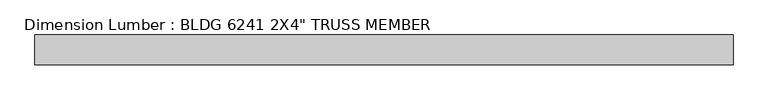
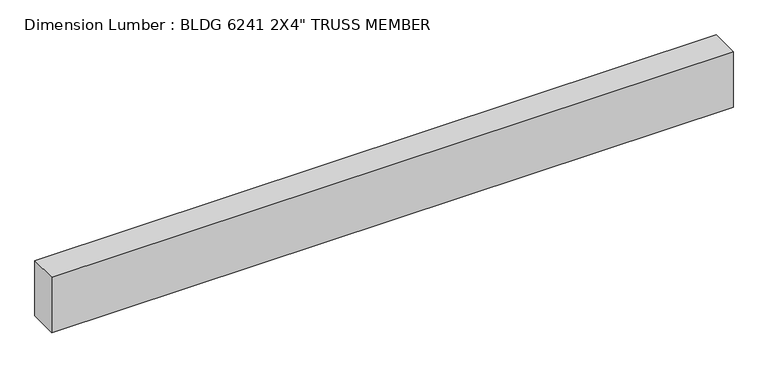
"""IFC4 building model written with IfcOpenShell, lengths in millimetres: beam geometry."""

from ifc_helpers import new_model, si_unit, frame, origin, place, context, project, spatial, polyline, outline, extrude, source, transform, mapped, element, save


def beam_af5d22dc(model_context):
    return source(origin(), model_context, "Body", "SweptSolid", [
        extrude(outline(polyline([(571.5, 25.4), (571.5, -25.4), (-609.6, -25.4), (-609.6, 25.4), (571.5, 25.4)])), frame((0.0, 0.0, -50.8), z_axis=(0.0, 0.0, 1.0), x_axis=(1.0, 0.0, 0.0)), (0.0, 0.0, 1.0), 101.6),
    ])


if __name__ == "__main__":
    model = new_model("IFC4")
    model_context = context("Model", 3, world=origin())
    ifc_project = project(units=[si_unit("LENGTHUNIT", "METRE", prefix="MILLI")], contexts=[model_context])
    site = spatial("IfcSite", under=ifc_project)
    building = spatial("IfcBuilding", under=site)
    placement = place(None, origin())
    beam_shape = beam_af5d22dc(model_context)
    element("IfcBeam", 1, ObjectType="Dimension Lumber : BLDG 6241 2X4\" TRUSS MEMBER", at=placement, inside=building, context=model_context, shape_type="MappedRepresentation", body=[
        mapped(beam_shape, transform((0.0, 0.0, 0.0), x_axis=(1.0, 0.0, 0.0), y_axis=(0.0, 1.0, 0.0), z_axis=(0.0, 0.0, 1.0))),
    ])
    save(model, "model.ifc")

# Revit data of these elements
# Type "Dimension Lumber : BLDG 6241 2X4\" TRUSS MEMBER"
#   Assembly Code = "B10"
#   A = 0.273472 SF
#   Length [instance default] = 5' - 0"
#   b = 0' - 2"
#   d = 0' - 4"
#   Structural Material [instance default] = Softwood, Lumber
# Element 1 (IfcBeam, "Dimension Lumber : BLDG 6241 2X4\" TRUSS MEMBER")
#   Materials on its faces: "Softwood, Lumber"
# Materials
#   "Softwood, Lumber": class "Wood", colour RGB 223 192 134, transparency 0, Description = "Pinus Echinata", Cost = 0
